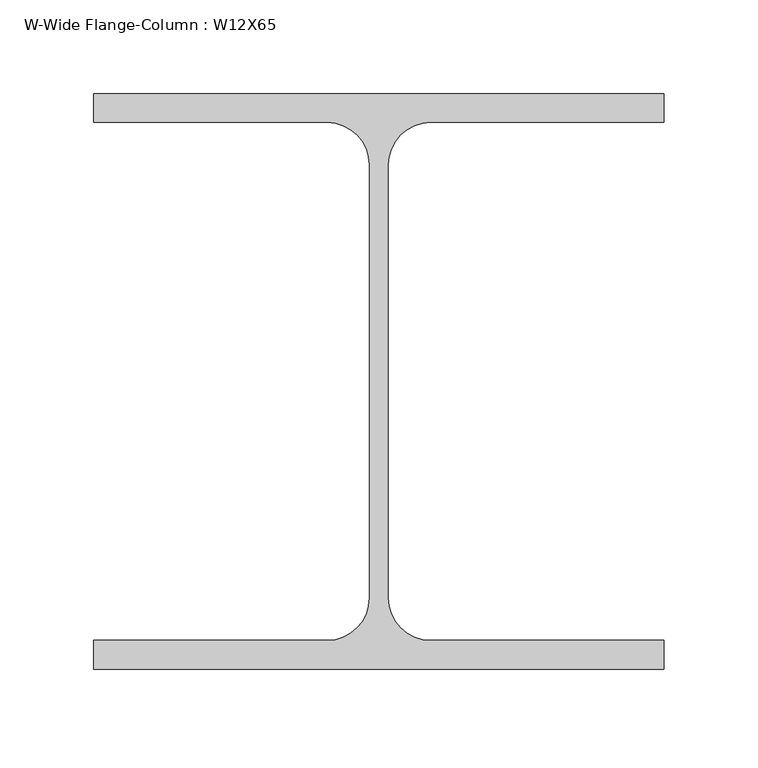
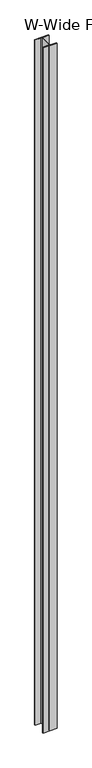
"""IFC4 building model written with IfcOpenShell, lengths in millimetres: column geometry, W-Wide Flange-Column : W12X65."""

import ifcopenshell
import ifcopenshell.guid

model = None  # the IFC model being written
_history = None  # IfcOwnerHistory: only IFC2X3 demands one
_inside = {}  # id of a spatial element -> (the spatial element, [elements in it])
_under = {}  # id of a project, library or spatial element -> (it, [spatial elements below it])
_declared = {}  # id of a project -> (the project, [libraries it declares])
_typed = {}  # id of a type object -> (the type object, [elements of that type])
_made_of = {}  # id of a material, layer set ... -> (it, [elements and type objects made of it])


def new_model(schema):
    """Start an empty IFC model of exactly this schema.

    Asked for "IFC4X3", IfcOpenShell would pick the latest addendum, in which some entities
    have other attributes; the version numbers below select the first issue.
    IFC2X3 requires an IfcOwnerHistory on every rooted entity: one is made here for all.
    """
    global model, _history
    if schema == "IFC4X3":
        model = ifcopenshell.file(schema_version=(4, 3, 0, 0))
    else:
        model = ifcopenshell.file(schema=schema)
    _inside.clear()
    _under.clear()
    _declared.clear()
    _typed.clear()
    _made_of.clear()
    _history = None
    if model.schema == "IFC2X3":
        org = make("IfcOrganization", Name="unknown")
        user = make(
            "IfcPersonAndOrganization",
            ThePerson=make("IfcPerson", FamilyName="unknown"),
            TheOrganization=org,
        )
        app = make(
            "IfcApplication",
            ApplicationDeveloper=org,
            Version="unknown",
            ApplicationFullName="unknown",
            ApplicationIdentifier="unknown",
        )
        _history = make(
            "IfcOwnerHistory",
            OwningUser=user,
            OwningApplication=app,
            ChangeAction="ADDED",
            CreationDate=0,
        )
    return model


def make(cls, **values):
    """One entity of the class cls with the attributes given. An attribute that is None is left unset."""
    return model.create_entity(
        cls, **{name: value for name, value in values.items() if value is not None}
    )


def rooted(cls, **values):
    """An entity with a GlobalId (a new one), such as an element, a storey or a relation."""
    return make(cls, GlobalId=ifcopenshell.guid.new(), OwnerHistory=_history, **values)


def si_unit(unit_type, name, prefix=None):
    """IfcSIUnit, for example si_unit("LENGTHUNIT", "METRE", prefix="MILLI")."""
    return make("IfcSIUnit", UnitType=unit_type, Prefix=prefix, Name=name)


def assignment(units):
    """IfcUnitAssignment: the units of a project."""
    return None if units is None else make("IfcUnitAssignment", Units=units)


def point(xyz):
    """IfcCartesianPoint."""
    return None if xyz is None else make("IfcCartesianPoint", Coordinates=xyz)


def direction(xyz):
    """IfcDirection."""
    return None if xyz is None else make("IfcDirection", DirectionRatios=xyz)


def frame(location, z_axis=None, x_axis=None):
    """IfcAxis2Placement3D, a coordinate frame: its origin and axes. An axis left out is left unset."""
    return make(
        "IfcAxis2Placement3D",
        Location=point(location),
        Axis=direction(z_axis),
        RefDirection=direction(x_axis),
    )


def frame_2d(location, x_axis=None):
    """IfcAxis2Placement2D, a coordinate frame in the plane: its origin and x axis."""
    return make(
        "IfcAxis2Placement2D", Location=point(location), RefDirection=direction(x_axis)
    )


def origin():
    """The frame at (0, 0, 0) with its axes left unset."""
    return frame((0.0, 0.0, 0.0))


def place(relative_to, where):
    """IfcLocalPlacement: puts the frame where relative to a parent placement (None: the world)."""
    return make(
        "IfcLocalPlacement", PlacementRelTo=relative_to, RelativePlacement=where
    )


def context(
    kind, dimensions, precision=None, world=None, true_north=None, identifier=None
):
    """IfcGeometricRepresentationContext, for example the 3D "Model" context."""
    return make(
        "IfcGeometricRepresentationContext",
        ContextIdentifier=identifier,
        ContextType=kind,
        CoordinateSpaceDimension=dimensions,
        Precision=precision,
        WorldCoordinateSystem=world,
        TrueNorth=true_north,
    )


def project(units=None, contexts=None):
    """IfcProject with its units and contexts."""
    return rooted(
        "IfcProject",
        Name="project",
        RepresentationContexts=contexts,
        UnitsInContext=assignment(units),
    )


def spatial(cls, under=None, at=None, **own):
    """A site, building, storey or space (cls), placed at a placement, below another one or the project."""
    s = rooted(cls, ObjectPlacement=at, **own)
    if under is not None:
        _under.setdefault(under.id(), (under, []))[1].append(s)
    return s


def polyline(points):
    """IfcPolyline through the points."""
    return make("IfcPolyline", Points=[point(p) for p in points])


def circle_curve(where, radius):
    """IfcCircle in the frame where."""
    return make("IfcCircle", Position=where, Radius=radius)


def trimmed(basis, trim1, trim2, sense, master):
    """IfcTrimmedCurve: the piece of a basis curve between two trims."""
    return make(
        "IfcTrimmedCurve",
        BasisCurve=basis,
        Trim1=trim1,
        Trim2=trim2,
        SenseAgreement=sense,
        MasterRepresentation=master,
    )


def segment(curve, same_sense, transition):
    """IfcCompositeCurveSegment."""
    return make(
        "IfcCompositeCurveSegment",
        Transition=transition,
        SameSense=same_sense,
        ParentCurve=curve,
    )


def composite_curve(segments, self_intersect=None):
    """IfcCompositeCurve: segments joined end to end."""
    return make("IfcCompositeCurve", Segments=segments, SelfIntersect=self_intersect)


def outline(outer, holes=None, kind="AREA"):
    """IfcArbitraryClosedProfileDef: a profile drawn as a closed curve; with holes, ...WithVoids."""
    if holes is None:
        return make("IfcArbitraryClosedProfileDef", ProfileType=kind, OuterCurve=outer)
    return make(
        "IfcArbitraryProfileDefWithVoids",
        ProfileType=kind,
        OuterCurve=outer,
        InnerCurves=holes,
    )


def extrude(swept, where, along, depth):
    """IfcExtrudedAreaSolid: the profile swept, set in the frame where, extruded along a direction by depth."""
    return make(
        "IfcExtrudedAreaSolid",
        SweptArea=swept,
        Position=where,
        ExtrudedDirection=direction(along),
        Depth=depth,
    )


def shape(context_of_items, identifier, shape_type, items):
    """IfcShapeRepresentation: the items that make up one representation, for example the "Body"."""
    return make(
        "IfcShapeRepresentation",
        ContextOfItems=context_of_items,
        RepresentationIdentifier=identifier,
        RepresentationType=shape_type,
        Items=items,
    )


def source(mapping_origin, context_of_items, identifier, shape_type, items):
    """IfcRepresentationMap: a shape defined once, which mapped items show again and again."""
    return make(
        "IfcRepresentationMap",
        MappingOrigin=mapping_origin,
        MappedRepresentation=shape(context_of_items, identifier, shape_type, items),
    )


def transform(
    local_origin,
    x_axis=None,
    y_axis=None,
    z_axis=None,
    scale=None,
    scale2=None,
    scale3=None,
    uniform=True,
):
    """IfcCartesianTransformationOperator3D, or its non-uniform kind. x_axis, y_axis, z_axis: its Axis1, 2, 3."""
    if uniform:
        return make(
            "IfcCartesianTransformationOperator3D",
            Axis1=direction(x_axis),
            Axis2=direction(y_axis),
            LocalOrigin=point(local_origin),
            Scale=scale,
            Axis3=direction(z_axis),
        )
    return make(
        "IfcCartesianTransformationOperator3DnonUniform",
        Axis1=direction(x_axis),
        Axis2=direction(y_axis),
        LocalOrigin=point(local_origin),
        Scale=scale,
        Axis3=direction(z_axis),
        Scale2=scale2,
        Scale3=scale3,
    )


def mapped(mapping_source, mapping_target):
    """IfcMappedItem: shows the shape of a source again, moved by a transform."""
    return make(
        "IfcMappedItem", MappingSource=mapping_source, MappingTarget=mapping_target
    )


def made_of(thing, what):
    """Note that an element or type object is made of a material, layer set ...; save() writes the relation."""
    if what is not None:
        _made_of.setdefault(what.id(), (what, []))[1].append(thing)
    return thing


def element(
    cls,
    number,
    at=None,
    inside=None,
    cuts=None,
    type_object=None,
    material=None,
    context=None,
    identifier="Body",
    shape_type=None,
    held_by="IfcProductDefinitionShape",
    body=None,
    shapes=None,
    **own,
):
    """One element of the class cls, such as IfcWall. Its Tag is "e" and its number.

    at: its placement. inside: the storey or other place that contains it. cuts: it is an
    opening in that element (IfcRelVoidsElement). A single representation is given by context,
    identifier, shape_type and body (its items); several are given by shapes. held_by: the class
    of the entity that holds the representations. save() writes the other relations.
    """
    e = rooted(cls, Tag="e%d" % number, ObjectPlacement=at, **own)
    if body is not None:
        shapes = [shape(context, identifier, shape_type, body)]
    if shapes is not None:
        e.Representation = make(held_by, Representations=shapes)
    if inside is not None:
        _inside.setdefault(inside.id(), (inside, []))[1].append(e)
    if cuts is not None:
        rooted(
            "IfcRelVoidsElement", RelatingBuildingElement=cuts, RelatedOpeningElement=e
        )
    if type_object is not None:
        _typed.setdefault(type_object.id(), (type_object, []))[1].append(e)
    return made_of(e, material)


def aggregate(whole, parts):
    """IfcRelAggregates: a whole, such as a stair, and the parts it consists of."""
    return rooted("IfcRelAggregates", RelatingObject=whole, RelatedObjects=parts)


def save(model, path):
    """Write the relations noted so far, then the file.

    IfcRelAggregates (storeys below a building ...), IfcRelContainedInSpatialStructure (elements
    in a storey), IfcRelDefinesByType, IfcRelAssociatesMaterial and IfcRelDeclares: one each for
    every whole, place, type object, material and project.
    """
    for whole, parts in _under.values():
        aggregate(whole, parts)
    for where, things in _inside.values():
        rooted(
            "IfcRelContainedInSpatialStructure",
            RelatedElements=things,
            RelatingStructure=where,
        )
    for kind, things in _typed.values():
        rooted("IfcRelDefinesByType", RelatedObjects=things, RelatingType=kind)
    for what, things in _made_of.values():
        rooted("IfcRelAssociatesMaterial", RelatedObjects=things, RelatingMaterial=what)
    for by, libraries in _declared.values():
        rooted("IfcRelDeclares", RelatingContext=by, RelatedDefinitions=libraries)
    model.write(path)


def w_wide_flange_column_w12x65_0830fbe6(model_context):
    return source(origin(), model_context, "Body", "SweptSolid", [
        extrude(outline(composite_curve([segment(polyline([(152.4, 153.67), (152.4, 138.303), (27.686, 138.303)]), True, "CONTINUOUS"), segment(trimmed(circle_curve(frame_2d((27.686, 115.57)), 22.733), [point((27.686, 138.303))], [point((4.953, 115.57))], True, "CARTESIAN"), True, "CONTINUOUS"), segment(polyline([(4.953, 115.57), (4.953, -115.57)]), True, "CONTINUOUS"), segment(trimmed(circle_curve(frame_2d((27.686, -115.57)), 22.733), [point((4.953, -115.57))], [point((27.686, -138.303))], True, "CARTESIAN"), True, "CONTINUOUS"), segment(polyline([(27.686, -138.303), (152.4, -138.303), (152.4, -153.67), (-152.4, -153.67), (-152.4, -138.303), (-27.686, -138.303)]), True, "CONTINUOUS"), segment(trimmed(circle_curve(frame_2d((-27.686, -115.57)), 22.733), [point((-27.686, -138.303))], [point((-4.953, -115.57))], True, "CARTESIAN"), True, "CONTINUOUS"), segment(polyline([(-4.953, -115.57), (-4.953, 115.57)]), True, "CONTINUOUS"), segment(trimmed(circle_curve(frame_2d((-27.686, 115.57)), 22.733), [point((-4.953, 115.57))], [point((-27.686, 138.303))], True, "CARTESIAN"), True, "CONTINUOUS"), segment(polyline([(-27.686, 138.303), (-152.4, 138.303), (-152.4, 153.67), (152.4, 153.67)]), True, "CONTINUOUS")], self_intersect=False)), frame((0.0, 0.0, 11849.1), z_axis=(0.0, 0.0, 1.0), x_axis=(1.0, 0.0, 0.0)), (0.0, 0.0, 1.0), 15735.3),
    ])


if __name__ == "__main__":
    model = new_model("IFC4")
    model_context = context("Model", 3, world=origin())
    ifc_project = project(units=[si_unit("LENGTHUNIT", "METRE", prefix="MILLI")], contexts=[model_context])
    site = spatial("IfcSite", under=ifc_project)
    building = spatial("IfcBuilding", under=site)
    placement = place(None, origin())
    w_wide_flange_column_w12x65_shape = w_wide_flange_column_w12x65_0830fbe6(model_context)
    element("IfcColumn", 1, ObjectType="W-Wide Flange-Column : W12X65", at=placement, inside=building, context=model_context, shape_type="MappedRepresentation", body=[
        mapped(w_wide_flange_column_w12x65_shape, transform((0.0, 0.0, 0.0), x_axis=(1.0, 0.0, 0.0), y_axis=(0.0, 1.0, 0.0), z_axis=(0.0, 0.0, 1.0))),
    ])
    save(model, "model.ifc")

# Revit data of these elements
# Type "W-Wide Flange-Column : W12X65"
#   Assembly Code = "B10"
#   W = 65
#   bf = 1' - 0"
#   d = 1' - 0.1"
#   k = 0' - 1 1/2"
#   kr = 0' - 0.895"
#   tf = 0' - 0.605"
#   tw = 0' - 0.39"
#   A = 0.132639 SF
#   Structural Material [instance default] = Steel ASTM A992
# Element 1 (IfcColumn, "W-Wide Flange-Column : W12X65")
#   Materials on its faces: "Steel ASTM A992"
# Materials
#   "Steel ASTM A992": class "Metal", colour RGB 199 199 199, transparency 0, Description = "Structural steel 50ksi", Cost = 0
